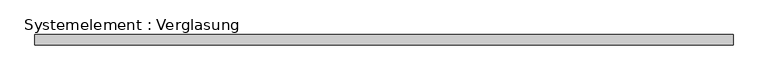
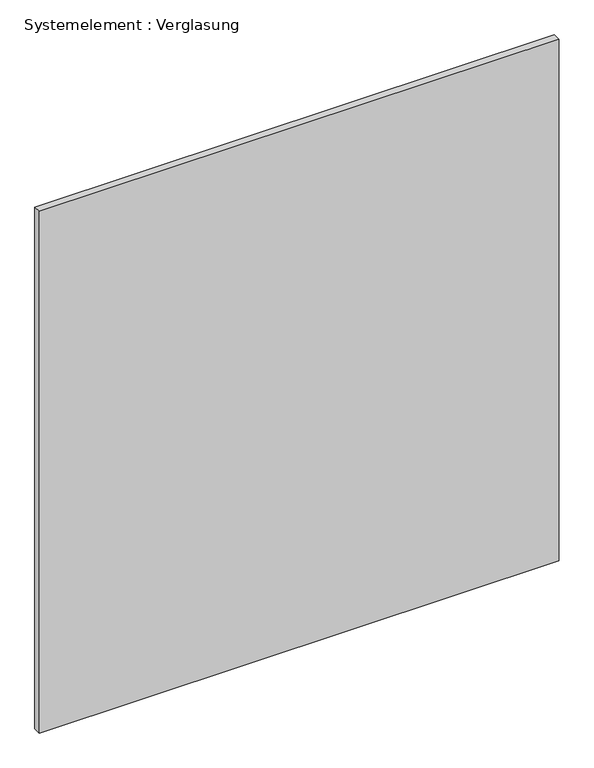
"""IFC4 building model written with IfcOpenShell, lengths in millimetres: plate geometry, Systemelement : Verglasung."""

from ifc_helpers import new_model, si_unit, origin, origin_with_axes, place, context, project, spatial, polyline, outline, extrude, source, transform, mapped, element, save


def systemelement_verglasung_12e0d43f(model_context):
    return source(origin(), model_context, "Body", "SweptSolid", [
        extrude(outline(polyline([(1025.0000002, -15.0), (-1025.0000002, -15.0), (-1025.0000002, 15.0), (1025.0000002, 15.0), (1025.0000002, -15.0)])), origin_with_axes(), (0.0, 0.0, 1.0), 2174.8398838),
    ])


if __name__ == "__main__":
    model = new_model("IFC4")
    model_context = context("Model", 3, world=origin())
    ifc_project = project(units=[si_unit("LENGTHUNIT", "METRE", prefix="MILLI")], contexts=[model_context])
    site = spatial("IfcSite", under=ifc_project)
    building = spatial("IfcBuilding", under=site)
    placement = place(None, origin())
    systemelement_verglasung_shape = systemelement_verglasung_12e0d43f(model_context)
    element("IfcPlate", 1, ObjectType="Systemelement : Verglasung", at=placement, inside=building, context=model_context, shape_type="MappedRepresentation", body=[
        mapped(systemelement_verglasung_shape, transform((0.0, 0.0, 0.0), x_axis=(1.0, 0.0, 0.0), y_axis=(0.0, 1.0, 0.0), z_axis=(0.0, 0.0, 1.0))),
    ])
    save(model, "model.ifc")

# Revit data of these elements
# Type "Systemelement : Verglasung"
#   Construction Type Id = "GSP4R"
#   Analytic Construction = "1/8 Zoll Pilkington-Verglasung einfach"
#   Visual Light Transmittance = 0.9
#   Solar Heat Gain Coefficient = 0.86
#   Heat Transfer Coefficient (U) = 6.7069 W/(m²·K)
# Element 1 (IfcPlate, "Systemelement : Verglasung")
#   Materials on its faces: "Glas"
# Materials
#   "Glas": class "Glas", colour RGB 0 0 255, transparency 0.75, Comments = "Render-Darstellung nicht aktualisiert ", Cost = 0
